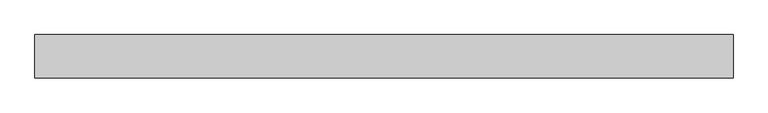
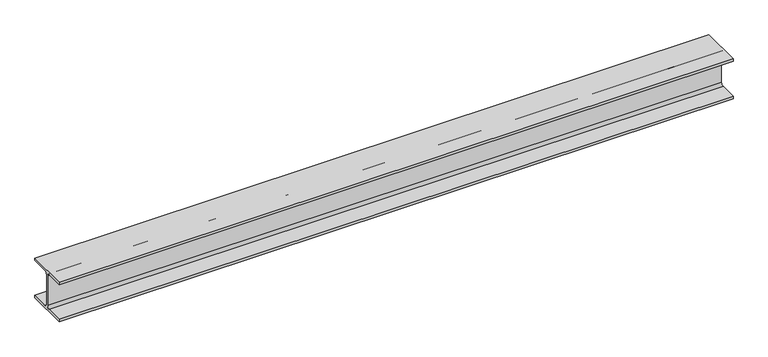
"""IFC4 building model written with IfcOpenShell, lengths in millimetres: beam geometry, 0912_Steel Framing_H-KSD3502 : H_SB_ASB_H-200x200x8x12."""

from ifc_helpers import new_model, si_unit, point, frame, frame_2d, origin, place, context, project, spatial, polyline, circle_curve, trimmed, segment, composite_curve, outline, extrude, source, transform, mapped, element, save


def beam_881e6142(model_context):
    return source(origin(), model_context, "Body", "SweptSolid", [
        extrude(outline(composite_curve([segment(polyline([(100.0, -88.0), (100.0, -100.0), (-100.0, -100.0), (-100.0, -88.0), (-17.0, -88.0)]), True, "CONTINUOUS"), segment(trimmed(circle_curve(frame_2d((-17.0, -75.0)), 13.0), [point((-17.0, -88.0))], [point((-4.0, -75.0))], True, "CARTESIAN"), True, "CONTINUOUS"), segment(polyline([(-4.0, -75.0), (-4.0, 75.0)]), True, "CONTINUOUS"), segment(trimmed(circle_curve(frame_2d((-17.0, 75.0)), 13.0), [point((-4.0, 75.0))], [point((-17.0, 88.0))], True, "CARTESIAN"), True, "CONTINUOUS"), segment(polyline([(-17.0, 88.0), (-100.0, 88.0), (-100.0, 100.0), (100.0, 100.0), (100.0, 88.0), (17.0, 88.0)]), True, "CONTINUOUS"), segment(trimmed(circle_curve(frame_2d((17.0, 75.0)), 13.0), [point((17.0, 88.0))], [point((4.0, 75.0))], True, "CARTESIAN"), True, "CONTINUOUS"), segment(polyline([(4.0, 75.0), (4.0, -75.0)]), True, "CONTINUOUS"), segment(trimmed(circle_curve(frame_2d((17.0, -75.0)), 13.0), [point((4.0, -75.0))], [point((17.0, -88.0))], True, "CARTESIAN"), True, "CONTINUOUS"), segment(polyline([(17.0, -88.0), (100.0, -88.0)]), True, "CONTINUOUS")], self_intersect=False)), frame((-1563.5376228, 0.0, 0.0), z_axis=(1.0, 0.0, 0.0), x_axis=(0.0, 1.0, 0.0)), (0.0, 0.0, 1.0), 3211.1247957),
    ])


if __name__ == "__main__":
    model = new_model("IFC4")
    model_context = context("Model", 3, world=origin())
    ifc_project = project(units=[si_unit("LENGTHUNIT", "METRE", prefix="MILLI")], contexts=[model_context])
    site = spatial("IfcSite", under=ifc_project)
    building = spatial("IfcBuilding", under=site)
    placement = place(None, origin())
    beam_shape = beam_881e6142(model_context)
    element("IfcBeam", 1, ObjectType="0912_Steel Framing_H-KSD3502 : H_SB_ASB_H-200x200x8x12", at=placement, inside=building, context=model_context, shape_type="MappedRepresentation", body=[
        mapped(beam_shape, transform((0.0, 0.0, 0.0), x_axis=(1.0, 0.0, 0.0), y_axis=(0.0, 1.0, 0.0), z_axis=(0.0, 0.0, 1.0))),
    ])
    save(model, "model.ifc")

# Revit data of these elements
# Type "0912_Steel Framing_H-KSD3502 : H_SB_ASB_H-200x200x8x12"
#   H_WM Code_1 = "S01AA002-00001 | Main Steel Structure Fabrication Work | Shelter/Building | Medium Steel - Standard (90KG/M>Weight≥30KG/M) | Material: (   )"
#   H_WM Code_2 = "S03AA028-00001 | Main Steel Structure Erection Work | Shelter/Building | Medium Steel (90KG/M>Weight≥30KG/M) | Material: (   )"
#   H_WM Code_3 = "S01AA010-00001 | Main Steel Structure Fabrication Work | Shelter/Building | Steel Painting/Coating | for Non-Fireproofed Steel Surface, Surface Preparation, Primer, Second & Final Coat | Material: (   )"
#   H_Q'ty Cal Type Tag = "SB-Q2"
#   Width = 20.0 cm
#   Web Thickness = 0.8 cm
#   Web Fillet = 1.3 cm
#   Warping Constant = 141000.0 cm⁶
#   W = 0
#   Torsional Moment of Inertia = 26.2485 cm⁴
#   Section Area = 63.53 cm²
#   Plastic Modulus weak axis = 244.0 cm³
#   Plastic Modulus strong axis = 525.0 cm³
#   Perimeter = 1.16 m²/m
#   Nominal Weight = 49.90 kgf/m
#   Moment of Inertia weak axis = 1600.00 cm⁴
#   Moment of Inertia strong axis = 4720.00 cm⁴
#   Height = 20.0 cm
#   Flange Thickness = 1.2 cm
#   Elastic Modulus weak axis = 160.0 cm³
#   Elastic Modulus strong axis = 472.0 cm³
#   Centroid Vertical = 10.0 cm
#   Centroid Horizontal = 10.0 cm
#   Ix = 47200000
#   Length [instance default] = 1.5240 m
#   Zx = 525000
#   b = 0.2000 m
#   h = 0.2000 m
#   r = 0.0130 m
#   s = 0.0080 m
#   t = 0.0120 m
#   A = 0.006353 m²
#   Structural Material [instance default] = Steel, 45-345
#   Assembly Code = ""
# Element 1 (IfcBeam, "0912_Steel Framing_H-KSD3502 : H_SB_ASB_H-200x200x8x12")
#   Structural Material = none
# Materials
#   "Steel, 45-345": class "Metal", colour RGB 189 187 185, transparency 0, Description = "Steel 345 MPa", Cost = 0
